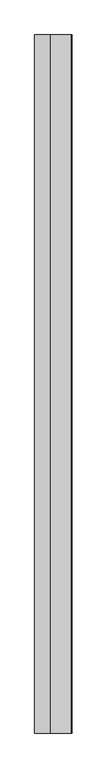
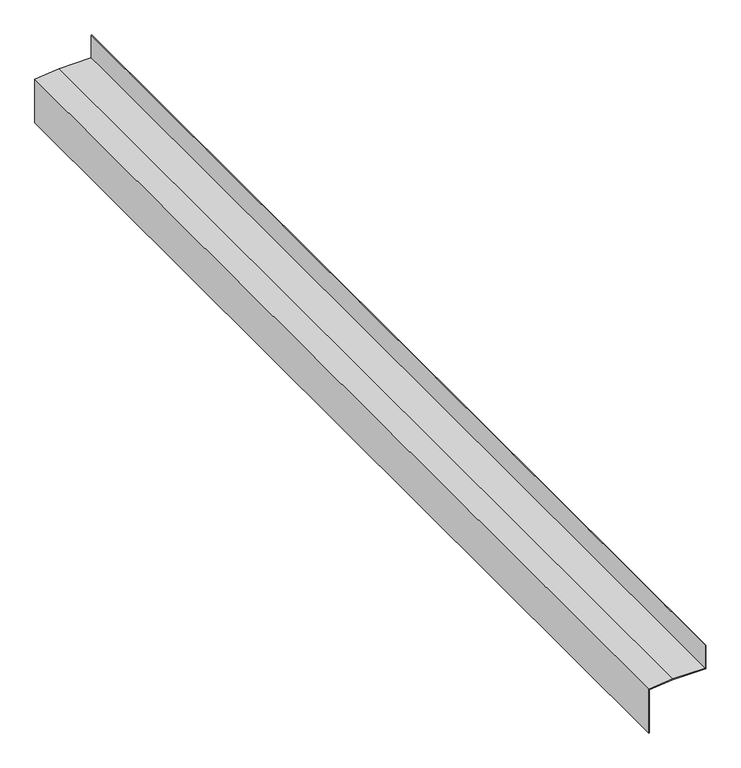
"""IFC4 building model written with IfcOpenShell, lengths in millimetres: proxy geometry, Generic Models 7:Generic Models 1:7:Generic Models 1:7 : Generic Models 7:Generic Models 1:337419:11 : Generic Models 7:Generic Models 1:7:Generic Models 1:7 : Generic Models 7:Generic Models 1:337419:315055."""

from ifc_helpers import new_model, si_unit, frame, origin, place, context, project, spatial, polyline, outline, extrude, source, transform, mapped, element, save


def generic_models_ade5a437(model_context):
    return source(origin(), model_context, "Body", "SweptSolid", [
        extrude(outline(polyline([(-83.6289841, 560223.1245374), (20.9992705, 560223.1245374), (26.9875, 560277.0537058), (26.9875, 560352.6118202), (83.9045258, 560352.6118202), (83.9045258, 560351.0243202), (28.575, 560351.0243202), (28.575, 560276.9658388), (22.420253, 560221.5370374), (-83.6289841, 560221.5370374), (-83.6289841, 560223.1245374)])), frame((0.0, -533090.1913841, 0.0), z_axis=(0.0, 1.0, 0.0), x_axis=(0.0, 0.0, 1.0)), (0.0, 0.0, 1.0), 2444.75),
    ])


if __name__ == "__main__":
    model = new_model("IFC4")
    model_context = context("Model", 3, world=origin())
    ifc_project = project(units=[si_unit("LENGTHUNIT", "METRE", prefix="MILLI")], contexts=[model_context])
    site = spatial("IfcSite", under=ifc_project)
    building = spatial("IfcBuilding", under=site)
    placement = place(None, origin())
    generic_models_shape = generic_models_ade5a437(model_context)
    element("IfcBuildingElementProxy", 1, Name="Generic Models 7:Generic Models 1:7:Generic Models 1:7 : Generic Models 7:Generic Models 1:337419:11 : Generic Models 7:Generic Models 1:7:Generic Models 1:7 : Generic Models 7:Generic Models 1:337419:315055", ObjectType="Generic Models 7:Generic Models 1:7:Generic Models 1:7 : Generic Models 7:Generic Models 1:337419:11 : Generic Models 7:Generic Models 1:7:Generic Models 1:7 : Generic Models 7:Generic Models 1:337419:315055", at=placement, inside=building, context=model_context, shape_type="MappedRepresentation", body=[
        mapped(generic_models_shape, transform((0.0, 0.0, 0.0), x_axis=(1.0, 0.0, 0.0), y_axis=(0.0, 1.0, 0.0), z_axis=(0.0, 0.0, 1.0))),
    ])
    save(model, "model.ifc")

# Revit data of these elements
# Type "Generic Models 7:Generic Models 1:7:Generic Models 1:7 : Generic Models 7:Generic Models 1:337419:11 : Generic Models 7:Generic Models 1:7:Generic Models 1:7 : Generic Models 7:Generic Models 1:337419:315055"
#   NameOverride = "Generic Models 7:Generic Models 1:7:Generic Models 1:7 : Generic Models 7:Generic Models 1:337419:315055"
#   ObjectTypeOverride = "Generic Models 1:7 : Generic Models 7:Generic Models 1:337419"
#   Reference = "Generic Models 1"
#   Tag = "315055"
# Element 1 (IfcBuildingElementProxy, "Generic Models 7:Generic Models 1:7:Generic Models 1:7 : Generic Models 7:Generic Models 1:337419:11 : Generic Models 7:Generic Models 1:7:Generic Models 1:7 : Generic Models 7:Generic Models 1:337419:315055")
#   Materials on its faces: "ANODIZED ALUM. FLASHING - MATCH STOREFRONT (ALIGN WITH OTHER WALL ASSEMBLIES)"
# Materials
#   "ANODIZED ALUM. FLASHING - MATCH STOREFRONT (ALIGN WITH OTHER WALL ASSEMBLIES)": class "Unassigned", colour RGB 210 209 208, transparency 0, Cost = 0
